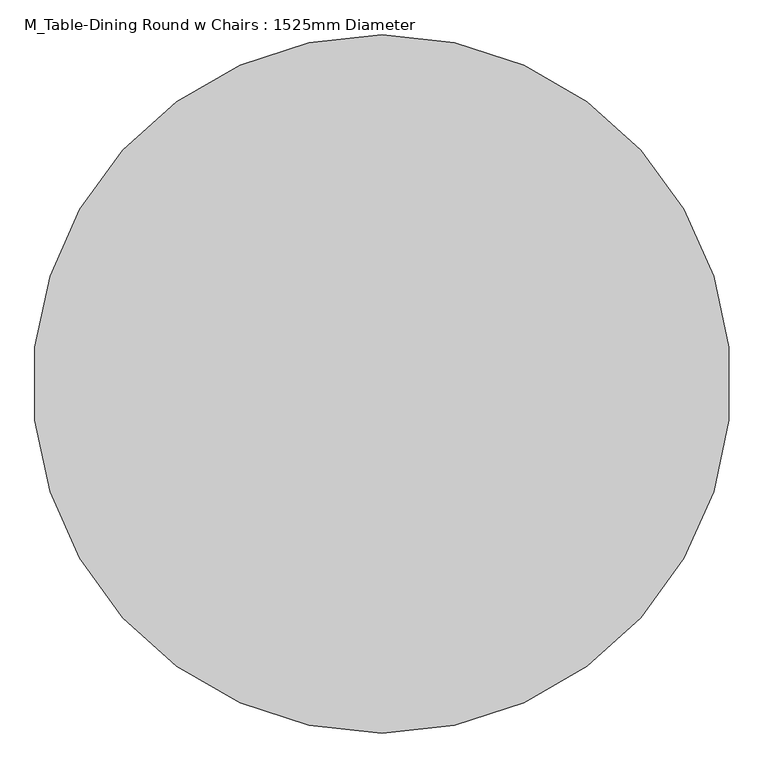
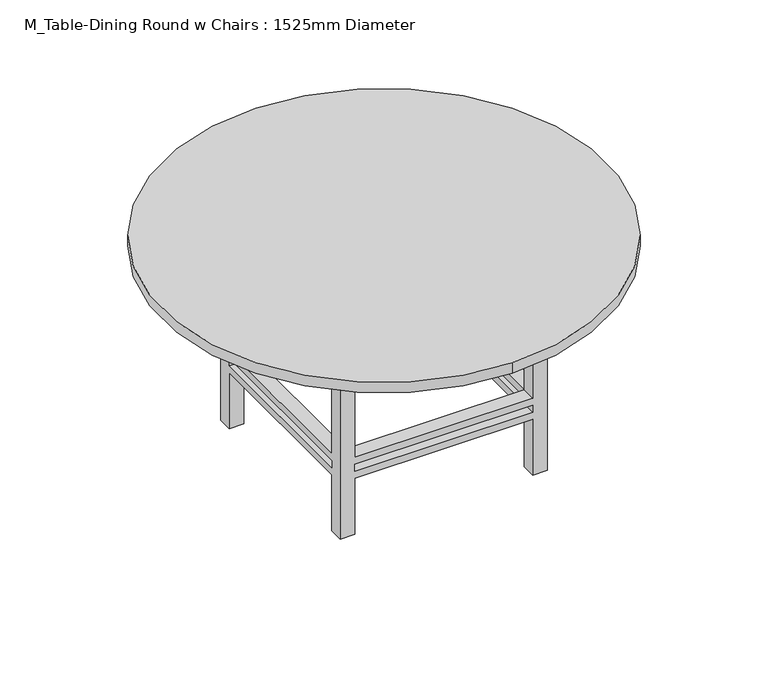
"""IFC4 building model written with IfcOpenShell, lengths in millimetres: furniture geometry, M_Table-Dining Round w Chairs : 1525mm Diameter."""

from ifc_helpers import new_model, si_unit, point, frame, frame_2d, origin, place, context, project, spatial, polyline, circle_curve, trimmed, segment, composite_curve, outline, extrude, faceted_brep, source, transform, mapped, element, save


def m_table_dining_round_w_chairs_1525mm_diameter_e8096f67(model_context):
    return source(origin(), model_context, "Body", "SolidModel", [
        faceted_brep([(-201.3680328, 170.9713115, 647.7), (-252.1680328, 170.9713115, 647.7), (-252.1680328, 120.1713115, 647.7), (-201.3680328, 120.1713115, 647.7), (408.7319672, 170.9713115, 647.7), (408.7319672, 120.1713115, 647.7), (459.5319672, 120.1713115, 647.7), (459.5319672, 170.9713115, 647.7), (408.7319672, -540.7286885, 647.7), (459.5319672, -540.7286885, 647.7), (459.5319672, -489.9286885, 647.7), (408.7319672, -489.9286885, 647.7), (-201.3680328, -540.7286885, 647.7), (-201.3680328, -489.9286885, 647.7), (-252.1680328, -489.9286885, 647.7), (-252.1680328, -540.7286885, 647.7), (-201.3680328, 170.9713115, 0.0), (-201.3680328, 120.1713115, 0.0), (-252.1680328, 120.1713115, 0.0), (-252.1680328, 170.9713115, 0.0), (408.7319672, 170.9713115, 0.0), (459.5319672, 170.9713115, 0.0), (459.5319672, 120.1713115, 0.0), (408.7319672, 120.1713115, 0.0), (408.7319672, -540.7286885, 0.0), (408.7319672, -489.9286885, 0.0), (459.5319672, -489.9286885, 0.0), (459.5319672, -540.7286885, 0.0), (-201.3680328, -540.7286885, 0.0), (-252.1680328, -540.7286885, 0.0), (-252.1680328, -489.9286885, 0.0), (-201.3680328, -489.9286885, 0.0), (-201.3680328, 170.9713115, 279.4), (408.7319672, 170.9713115, 279.4), (408.7319672, 170.9713115, 203.2), (-201.3680328, 170.9713115, 203.2), (408.7319672, 170.9713115, 228.6), (408.7319672, 170.9713115, 254.0), (-201.3680328, 170.9713115, 254.0), (-201.3680328, 170.9713115, 228.6), (-252.1680328, 120.1713115, 203.2), (-252.1680328, -489.9286885, 203.2), (-252.1680328, -489.9286885, 279.4), (-252.1680328, 120.1713115, 279.4), (-252.1680328, 120.1713115, 228.6), (-252.1680328, 120.1713115, 254.0), (-252.1680328, -489.9286885, 254.0), (-252.1680328, -489.9286885, 228.6), (-201.3680328, 120.1713115, 279.4), (-201.3680328, 120.1713115, 203.2), (-201.3680328, 120.1713115, 228.6), (-201.3680328, 120.1713115, 254.0), (408.7319672, 120.1713115, 279.4), (408.7319672, 120.1713115, 203.2), (408.7319672, 120.1713115, 228.6), (408.7319672, 120.1713115, 254.0), (459.5319672, 120.1713115, 279.4), (459.5319672, 120.1713115, 203.2), (459.5319672, 120.1713115, 228.6), (459.5319672, 120.1713115, 254.0), (459.5319672, -489.9286885, 279.4), (459.5319672, -489.9286885, 203.2), (459.5319672, -489.9286885, 228.6), (459.5319672, -489.9286885, 254.0), (408.7319672, -540.7286885, 279.4), (-201.3680328, -540.7286885, 279.4), (-201.3680328, -540.7286885, 203.2), (408.7319672, -540.7286885, 203.2), (-201.3680328, -540.7286885, 228.6), (-201.3680328, -540.7286885, 254.0), (408.7319672, -540.7286885, 254.0), (408.7319672, -540.7286885, 228.6), (408.7319672, -489.9286885, 279.4), (408.7319672, -489.9286885, 203.2), (408.7319672, -489.9286885, 228.6), (408.7319672, -489.9286885, 254.0), (-201.3680328, -489.9286885, 279.4), (-201.3680328, -489.9286885, 203.2), (-201.3680328, -489.9286885, 228.6), (-201.3680328, -489.9286885, 254.0)], [[[0, 1, 2, 3]], [[4, 5, 6, 7]], [[8, 9, 10, 11]], [[12, 13, 14, 15]], [[16, 17, 18, 19]], [[20, 21, 22, 23]], [[24, 25, 26, 27]], [[28, 29, 30, 31]], [[1, 0, 32, 33, 4, 7, 21, 20, 34, 35, 16, 19], [36, 37, 38, 39]], [[2, 1, 19, 18, 40, 41, 30, 29, 15, 14, 42, 43], [44, 45, 46, 47]], [[3, 2, 43, 48]], [[18, 17, 49, 40]], [[44, 50, 51, 45]], [[0, 3, 48, 32]], [[17, 16, 35, 49]], [[50, 39, 38, 51]], [[5, 4, 33, 52]], [[20, 23, 53, 34]], [[36, 54, 55, 37]], [[6, 5, 52, 56]], [[23, 22, 57, 53]], [[54, 58, 59, 55]], [[21, 7, 6, 56, 60, 10, 9, 27, 26, 61, 57, 22], [62, 63, 59, 58]], [[27, 9, 8, 64, 65, 12, 15, 29, 28, 66, 67, 24], [68, 69, 70, 71]], [[11, 10, 60, 72]], [[26, 25, 73, 61]], [[62, 74, 75, 63]], [[8, 11, 72, 64]], [[25, 24, 67, 73]], [[74, 71, 70, 75]], [[13, 12, 65, 76]], [[28, 31, 77, 66]], [[68, 78, 79, 69]], [[14, 13, 76, 42]], [[31, 30, 41, 77]], [[78, 47, 46, 79]], [[54, 74, 62, 58]], [[74, 78, 68, 71]], [[78, 50, 44, 47]], [[50, 54, 36, 39]], [[53, 49, 35, 34]], [[49, 77, 41, 40]], [[77, 73, 67, 66]], [[73, 53, 57, 61]], [[74, 54, 53, 73]], [[78, 74, 73, 77]], [[50, 78, 77, 49]], [[54, 50, 49, 53]], [[52, 72, 60, 56]], [[72, 76, 65, 64]], [[76, 48, 43, 42]], [[48, 52, 33, 32]], [[55, 51, 38, 37]], [[51, 79, 46, 45]], [[79, 75, 70, 69]], [[75, 55, 59, 63]], [[72, 52, 55, 75]], [[76, 72, 75, 79]], [[48, 76, 79, 51]], [[52, 48, 51, 55]]]),
        extrude(outline(polyline([(484.9319672, 196.3713115), (484.9319672, -566.1286885), (-277.5680328, -566.1286885), (-277.5680328, 196.3713115), (484.9319672, 196.3713115)]), holes=[polyline([(459.5319672, 170.9713115), (-252.1680328, 170.9713115), (-252.1680328, -540.7286885), (459.5319672, -540.7286885), (459.5319672, 170.9713115)])]), frame((0.0, 0.0, 647.7), z_axis=(0.0, 0.0, 1.0), x_axis=(1.0, 0.0, 0.0)), (0.0, 0.0, 1.0), 76.2),
        extrude(outline(composite_curve([segment(trimmed(circle_curve(frame_2d((103.6819672, -184.8786885)), 762.5), [point((103.6819672, -947.3786885))], [point((103.6819672, 577.6213115))], False, "CARTESIAN"), True, "CONTINUOUS"), segment(trimmed(circle_curve(frame_2d((103.6819672, -184.8786885)), 762.5), [point((103.6819672, 577.6213115))], [point((103.6819672, -947.3786885))], False, "CARTESIAN"), True, "CONTINUOUS")], self_intersect=False)), frame((0.0, 0.0, 723.9), z_axis=(0.0, 0.0, 1.0), x_axis=(1.0, 0.0, 0.0)), (0.0, 0.0, 1.0), 38.1),
    ])


if __name__ == "__main__":
    model = new_model("IFC4")
    model_context = context("Model", 3, world=origin())
    ifc_project = project(units=[si_unit("LENGTHUNIT", "METRE", prefix="MILLI")], contexts=[model_context])
    site = spatial("IfcSite", under=ifc_project)
    building = spatial("IfcBuilding", under=site)
    placement = place(None, origin())
    m_table_dining_round_w_chairs_1525mm_diameter_shape = m_table_dining_round_w_chairs_1525mm_diameter_e8096f67(model_context)
    element("IfcFurniture", 1, ObjectType="M_Table-Dining Round w Chairs : 1525mm Diameter", at=placement, inside=building, context=model_context, shape_type="MappedRepresentation", body=[
        mapped(m_table_dining_round_w_chairs_1525mm_diameter_shape, transform((0.0, 0.0, 0.0), x_axis=(1.0, 0.0, 0.0), y_axis=(0.0, 1.0, 0.0), z_axis=(0.0, 0.0, 1.0))),
    ])
    save(model, "model.ifc")

# Revit data of these elements
# Type "M_Table-Dining Round w Chairs : 1525mm Diameter"
#   Radius = 0.7625 m
#   Diameter = 1.525 m
#   Height = 0.762 m
#   Chairs = 6
#   Base Material = Pine
#   Top Material = Laminate, Linen, Matte
#   Default Elevation = 0
# Element 1 (IfcFurniture, "M_Table-Dining Round w Chairs : 1525mm Diameter")
#   Materials on its faces: "Pine", "Laminate, Linen, Matte"
# Materials
#   "Pine": class "Wood", colour RGB 223 192 134, transparency 0, Description = "Pinus Echinata", Cost = 0
#   "Laminate, Linen, Matte": class "Plastic", colour RGB 249 239 230, transparency 0, Description = "Plastic Laminate - Linen, Matte", Cost = 0
